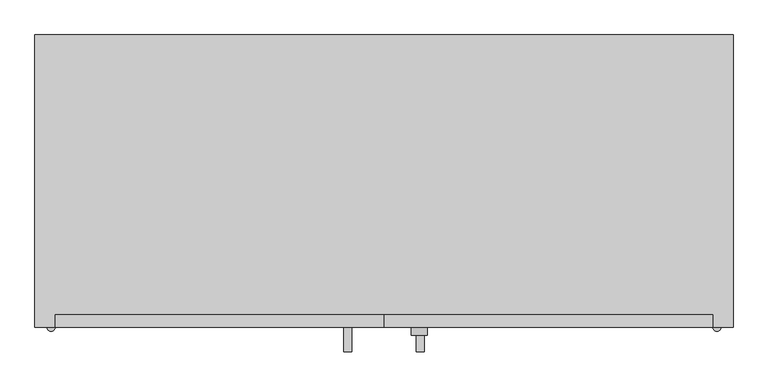
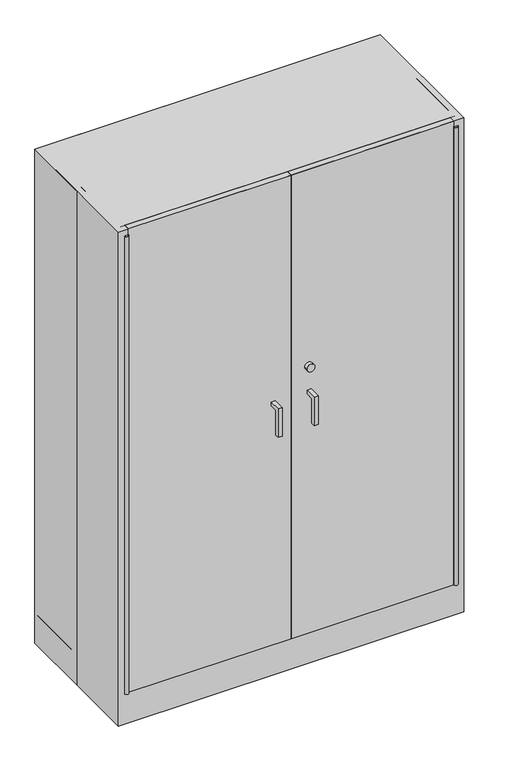
"""IFC4 building model written with IfcOpenShell, lengths in millimetres: proxy geometry, M2015 - Cabinet, Storage, Flammable, Freestanding : M2015 - Cabinet, Storage, Flammable, Freestanding."""

from ifc_helpers import new_model, si_unit, point, frame, frame_2d, origin, origin_with_axes, place, context, project, spatial, polyline, circle_curve, trimmed, segment, composite_curve, outline, extrude, source, transform, mapped, element, save


def specialty_equipment_634e261d(model_context):
    return source(origin(), model_context, "Body", "SweptSolid", [
        extrude(outline(composite_curve([segment(trimmed(circle_curve(frame_2d((994.2982536, 55.3458716)), 12.7), [point((994.2982536, 42.6458716))], [point((994.2982536, 68.0458716))], False, "CARTESIAN"), True, "CONTINUOUS"), segment(trimmed(circle_curve(frame_2d((994.2982536, 55.3458716)), 12.7), [point((994.2982536, 68.0458716))], [point((994.2982536, 42.6458716))], False, "CARTESIAN"), True, "CONTINUOUS")], self_intersect=False)), frame((0.0, -241.3, 0.0), z_axis=(0.0, 1.0, 0.0), x_axis=(0.0, 0.0, 1.0)), (0.0, 0.0, 1.0), 12.7),
        extrude(outline(polyline([(-266.7, 819.15), (-266.7, 914.4), (-228.6, 914.4), (-228.6, 901.7159299), (-254.0159299, 901.7159299), (-254.0159299, 831.8340701), (-254.0159299, 819.15), (-266.7, 819.15)])), frame((-63.2065288, 0.0, 0.0), z_axis=(1.0, 0.0, 0.0), x_axis=(0.0, 1.0, 0.0)), (0.0, 0.0, 1.0), 12.7),
        extrude(outline(polyline([(-266.7, 819.15), (-266.7, 914.4), (-228.6, 914.4), (-228.6, 901.7159299), (-254.0159299, 901.7159299), (-254.0159299, 831.8340701), (-254.0159299, 819.15), (-266.7, 819.15)])), frame((50.5065288, 0.0, 0.0), z_axis=(1.0, 0.0, 0.0), x_axis=(0.0, 1.0, 0.0)), (0.0, 0.0, 1.0), 12.7),
        extrude(outline(polyline([(514.35, -228.6), (0.0, -228.6), (0.0, -209.55), (514.35, -209.55), (514.35, -228.6)])), frame((0.0, 0.0, 101.6), z_axis=(0.0, 0.0, 1.0), x_axis=(1.0, 0.0, 0.0)), (0.0, 0.0, 1.0), 1549.4),
        extrude(outline(polyline([(0.0, -228.6), (-514.35, -228.6), (-514.35, -209.55), (0.0, -209.55), (0.0, -228.6)])), frame((0.0, 0.0, 101.6), z_axis=(0.0, 0.0, 1.0), x_axis=(1.0, 0.0, 0.0)), (0.0, 0.0, 1.0), 1549.4),
        extrude(outline(composite_curve([segment(trimmed(circle_curve(frame_2d((520.7, -228.6)), 6.35), [point((514.35, -228.6))], [point((527.05, -228.6))], False, "CARTESIAN"), True, "CONTINUOUS"), segment(trimmed(circle_curve(frame_2d((520.7, -228.6)), 6.35), [point((527.05, -228.6))], [point((514.35, -228.6))], False, "CARTESIAN"), True, "CONTINUOUS")], self_intersect=False)), frame((0.0, 0.0, 101.6), z_axis=(0.0, 0.0, 1.0), x_axis=(1.0, 0.0, 0.0)), (0.0, 0.0, 1.0), 1530.35),
        extrude(outline(composite_curve([segment(trimmed(circle_curve(frame_2d((-520.7, -228.6)), 6.35), [point((-514.35, -228.6))], [point((-527.05, -228.6))], False, "CARTESIAN"), True, "CONTINUOUS"), segment(trimmed(circle_curve(frame_2d((-520.7, -228.6)), 6.35), [point((-527.05, -228.6))], [point((-514.35, -228.6))], False, "CARTESIAN"), True, "CONTINUOUS")], self_intersect=False)), frame((0.0, 0.0, 101.6), z_axis=(0.0, 0.0, 1.0), x_axis=(1.0, 0.0, 0.0)), (0.0, 0.0, 1.0), 1530.35),
        extrude(outline(polyline([(-546.1, 228.6), (546.1, 228.6), (546.1, -228.6), (-546.1, -228.6), (-546.1, 0.0), (-546.1, 228.6)])), origin_with_axes(), (0.0, 0.0, 1.0), 1651.0),
        extrude(outline(polyline([(546.1, -196.85), (-546.1, -196.85), (-546.1, -177.8), (546.1, -177.8), (546.1, -196.85)])), origin_with_axes(), (0.0, 0.0, 1.0), 101.6),
        extrude(outline(polyline([(527.05, 228.6), (527.05, -209.55), (-527.05, -209.55), (-527.05, 228.6), (527.05, 228.6)])), frame((0.0, 0.0, 1631.95), z_axis=(0.0, 0.0, 1.0), x_axis=(1.0, 0.0, 0.0)), (0.0, 0.0, 1.0), 19.05),
        extrude(outline(polyline([(527.05, 209.55), (-527.05, 209.55), (-527.05, 228.6), (527.05, 228.6), (527.05, 209.55)])), origin_with_axes(), (0.0, 0.0, 1.0), 1631.95),
        extrude(outline(polyline([(527.05, -177.8), (527.05, 228.6), (546.1, 228.6), (546.1, -177.8), (527.05, -177.8)])), origin_with_axes(), (0.0, 0.0, 1.0), 101.6),
        extrude(outline(polyline([(527.05, -228.6), (527.05, 228.6), (546.1, 228.6), (546.1, -228.6), (527.05, -228.6)])), frame((0.0, 0.0, 101.6), z_axis=(0.0, 0.0, 1.0), x_axis=(1.0, 0.0, 0.0)), (0.0, 0.0, 1.0), 1549.4),
        extrude(outline(polyline([(-546.1, -177.8), (-546.1, 228.6), (-527.05, 228.6), (-527.05, -177.8), (-546.1, -177.8)])), origin_with_axes(), (0.0, 0.0, 1.0), 101.6),
        extrude(outline(polyline([(-546.1, -228.6), (-546.1, 228.6), (-527.05, 228.6), (-527.05, -228.6), (-546.1, -228.6)])), frame((0.0, 0.0, 101.6), z_axis=(0.0, 0.0, 1.0), x_axis=(1.0, 0.0, 0.0)), (0.0, 0.0, 1.0), 1549.4),
        extrude(outline(polyline([(527.05, 209.55), (527.05, -209.55), (-527.05, -209.55), (-527.05, 209.55), (527.05, 209.55)])), frame((0.0, 0.0, 101.6), z_axis=(0.0, 0.0, 1.0), x_axis=(1.0, 0.0, 0.0)), (0.0, 0.0, 1.0), 19.1166954),
    ])


if __name__ == "__main__":
    model = new_model("IFC4")
    model_context = context("Model", 3, world=origin())
    ifc_project = project(units=[si_unit("LENGTHUNIT", "METRE", prefix="MILLI")], contexts=[model_context])
    site = spatial("IfcSite", under=ifc_project)
    building = spatial("IfcBuilding", under=site)
    placement = place(None, origin())
    specialty_equipment_shape = specialty_equipment_634e261d(model_context)
    element("IfcBuildingElementProxy", 1, Name="M2015 - Cabinet, Storage, Flammable, Freestanding : M2015 - Cabinet, Storage, Flammable, Freestanding", ObjectType="M2015 - Cabinet, Storage, Flammable, Freestanding : M2015 - Cabinet, Storage, Flammable, Freestanding", at=placement, inside=building, context=model_context, shape_type="MappedRepresentation", body=[
        mapped(specialty_equipment_shape, transform((0.0, 0.0, 0.0), x_axis=(1.0, 0.0, 0.0), y_axis=(0.0, 1.0, 0.0), z_axis=(0.0, 0.0, 1.0))),
    ])
    save(model, "model.ifc")

# Revit data of these elements
# Type "M2015 - Cabinet, Storage, Flammable, Freestanding : M2015 - Cabinet, Storage, Flammable, Freestanding"
#   Watts2 = "0"
#   Watts1 = "0"
#   Unit_Issue = "EA"
#   UTIL_6_Misc = "-"
#   UTIL_5_NonMedGas = "-"
#   UTIL_4_MiscGas = "-"
#   UTIL_3_MedGas = "-"
#   UTIL_2_Elec = "-"
#   UTIL_1_WaterDrain = "-"
#   Nomenclature = "Cabinet, Storage, Flammable, Freestanding"
#   NSN = "7125"
#   Location [instance default] = ""
#   JSN = "M2015"
#   Fund_Source_VA = "-"
#   Fund_Source_Navy = "-"
#   Fund_Source_Army = "-"
#   Fund_Source_AF = "-"
#   ELEC_Volts2 = "0"
#   ELEC_Volts1 = "0"
#   ELEC_Phase2 = "0"
#   ELEC_Phase1 = "0"
#   ELEC_HertzSwitch = "0"
#   ELEC_HertzDependent = "0"
#   ELEC_Hertz = "0"
#   ELEC_Amps2 = "0"
#   ELEC_Amps1 = "0"
#   DetailDescription = "Freestanding flammable safety storage cabinet. Size as required. Unit is of all welded steel wall construction with vented grounding attachments, raised leak proof door sill and adjustable shelving. Equipped with swinging doors and built-in key lock. Designed for storage of flammable fluids. Complies with OSHA standards, is FM approved and designed IAW NFPA 30."
#   CAT_VA = "C"
#   CAT_Navy = "C"
#   CAT_IHS = "-"
#   CAT_Army = "C"
#   CAT_AF = "C"
#   BTUperhour = "0"
#   Weight_IP = 376
#   DIM_Width_IP = 3' - 7"
#   DIM_Height_IP = 5' - 5"
#   DIM_Depth_IP = 1' - 6"
#   Top Panel Material = none
#   Toe Panel Material = none
#   Side Panel Material = none
#   Shelf Panel Material = none
#   Drawer Front Material = none
#   Door Panel Material = none
#   Back Panel Material = none
#   Assembly Code = ""
# Element 1 (IfcBuildingElementProxy, "M2015 - Cabinet, Storage, Flammable, Freestanding : M2015 - Cabinet, Storage, Flammable, Freestanding")
#   Materials on its faces: "Default metal", "EquipSpace"
# Materials
#   "Default metal": class "Unassigned", colour RGB 204 204 204, transparency 0
#   "EquipSpace": class "Unassigned", colour RGB 221 217 195, transparency 0.5
